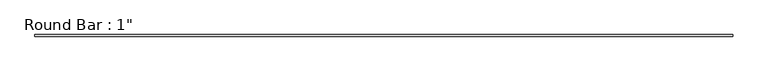
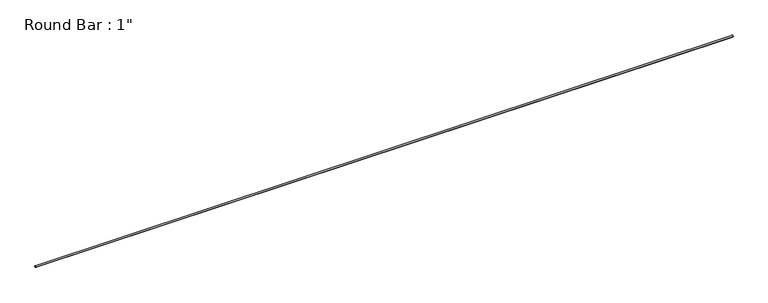
"""IFC4 building model written with IfcOpenShell, lengths in millimetres: member geometry."""

from ifc_helpers import new_model, si_unit, point, frame, origin, origin_2d, place, context, project, spatial, circle_curve, trimmed, segment, composite_curve, outline, extrude, source, transform, mapped, element, save


def member_59755b8b(model_context):
    return source(origin(), model_context, "Body", "SweptSolid", [
        extrude(outline(composite_curve([segment(trimmed(circle_curve(origin_2d(), 12.7), [point((12.7, 0.0))], [point((-12.7, 0.0))], False, "CARTESIAN"), True, "CONTINUOUS"), segment(trimmed(circle_curve(origin_2d(), 12.7), [point((-12.7, 0.0))], [point((12.7, 0.0))], False, "CARTESIAN"), True, "CONTINUOUS")], self_intersect=False)), frame((-5425.0253699, 0.0, 0.0), z_axis=(1.0, 0.0, 0.0), x_axis=(0.0, 1.0, 0.0)), (0.0, 0.0, 1.0), 10850.0507398),
    ])


if __name__ == "__main__":
    model = new_model("IFC4")
    model_context = context("Model", 3, world=origin())
    ifc_project = project(units=[si_unit("LENGTHUNIT", "METRE", prefix="MILLI")], contexts=[model_context])
    site = spatial("IfcSite", under=ifc_project)
    building = spatial("IfcBuilding", under=site)
    placement = place(None, origin())
    member_shape = member_59755b8b(model_context)
    element("IfcMember", 1, ObjectType="Round Bar : 1\"", at=placement, inside=building, context=model_context, shape_type="MappedRepresentation", body=[
        mapped(member_shape, transform((0.0, 0.0, 0.0), x_axis=(1.0, 0.0, 0.0), y_axis=(0.0, 1.0, 0.0), z_axis=(0.0, 0.0, 1.0))),
    ])
    save(model, "model.ifc")

# Revit data of these elements
# Type "Round Bar : 1\""
#   Assembly Code = "B10"
#   W = 0
#   Start Extension Calculation [instance default] = 10' - 0"
#   Start Extension [instance default] = -0' - 0 1/2"
#   End Extension Calculation [instance default] = 10' - 0"
#   End Extension [instance default] = -0' - 0 1/2"
#   Length [instance default] = 5' - 0"
#   d = 0' - 1"
#   A = 0 SF
#   Structural Material [instance default] = Metal - Steel - ASTM A36
# Element 1 (IfcMember, "Round Bar : 1\"")
#   Materials on its faces: "Metal - Steel - ASTM A36"
# Materials
#   "Metal - Steel - ASTM A36": class "Metal", colour RGB 199 199 199, transparency 0
